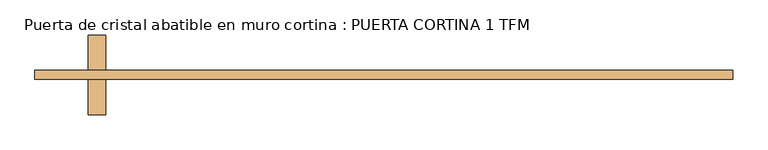
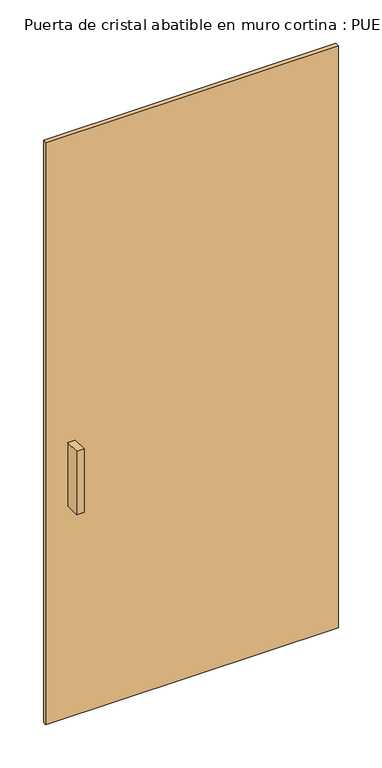
"""IFC4 building model written with IfcOpenShell, lengths in millimetres: door geometry, Puerta de cristal abatible en muro cortina : PUERTA CORTINA 1 TFM."""

from ifc_helpers import new_model, si_unit, frame, origin, origin_with_axes, place, context, project, spatial, polyline, outline, extrude, source, transform, mapped, element, save


def puerta_de_cristal_abatible_en_muro_cortina_puerta_cortina_1_2cb0721c(model_context):
    return source(origin(), model_context, "Body", "SweptSolid", [
        extrude(outline(polyline([(-398.4, -12.5), (-423.8, -12.5), (-423.8, 38.3), (-398.4, 38.3), (-398.4, -12.5)])), frame((0.0, 0.0, 762.0), z_axis=(0.0, 0.0, 1.0), x_axis=(1.0, 0.0, 0.0)), (0.0, 0.0, 1.0), 228.6),
        extrude(outline(polyline([(-423.8, 101.8), (-398.4, 101.8), (-398.4, 51.0), (-423.8, 51.0), (-423.8, 101.8)])), frame((0.0, 0.0, 762.0), z_axis=(0.0, 0.0, 1.0), x_axis=(1.0, 0.0, 0.0)), (0.0, 0.0, 1.0), 228.6),
        extrude(outline(polyline([(500.0, 51.0), (500.0, 38.3), (-500.0, 38.3), (-500.0, 51.0), (500.0, 51.0)])), origin_with_axes(), (0.0, 0.0, 1.0), 2100.0),
    ])


if __name__ == "__main__":
    model = new_model("IFC4")
    model_context = context("Model", 3, world=origin())
    ifc_project = project(units=[si_unit("LENGTHUNIT", "METRE", prefix="MILLI")], contexts=[model_context])
    site = spatial("IfcSite", under=ifc_project)
    building = spatial("IfcBuilding", under=site)
    placement = place(None, origin())
    puerta_de_cristal_abatible_en_muro_cortina_puerta_cortina_1_shape = puerta_de_cristal_abatible_en_muro_cortina_puerta_cortina_1_2cb0721c(model_context)
    element("IfcDoor", 1, ObjectType="Puerta de cristal abatible en muro cortina : PUERTA CORTINA 1 TFM", at=placement, inside=building, context=model_context, shape_type="MappedRepresentation", body=[
        mapped(puerta_de_cristal_abatible_en_muro_cortina_puerta_cortina_1_shape, transform((0.0, 0.0, 0.0), x_axis=(1.0, 0.0, 0.0), y_axis=(0.0, 1.0, 0.0), z_axis=(0.0, 0.0, 1.0))),
    ])
    save(model, "model.ifc")

# Revit data of these elements
# Type "Puerta de cristal abatible en muro cortina : PUERTA CORTINA 1 TFM"
#   Description = "Puerta vidrio muro cortina"
#   Type Mark = "P4"
#   Construction Type Id = "SGL"
#   Analytic Construction = "Ventanas grandes con acristalamiento simple"
#   Visual Light Transmittance = 0.9
#   Solar Heat Gain Coefficient = 0.86
#   Desfase = 0.051 m
#   Heat Transfer Coefficient (U) = 5.5617 W/(m²·K)
#   Define Thermal Properties by = 1
#   Function = 1
#   Material de cristalera = Vidrio
# Element 1 (IfcDoor, "Puerta de cristal abatible en muro cortina : PUERTA CORTINA 1 TFM")
#   Materials on its faces: "Metal - Aluminio", "Vidrio"
# Materials
#   "Vidrio": class "Vidrio", colour RGB 0 128 192, transparency 0.75, Description = "Vidrio de cal sodada", Cost = 0
#   "Metal - Aluminio": class "Metal", colour RGB 247 247 247, transparency 0
